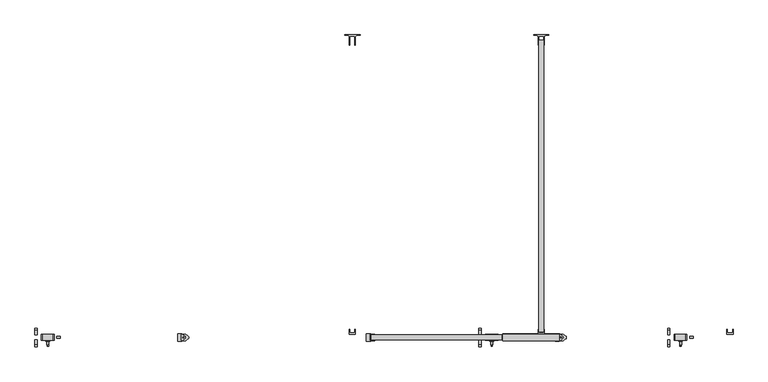
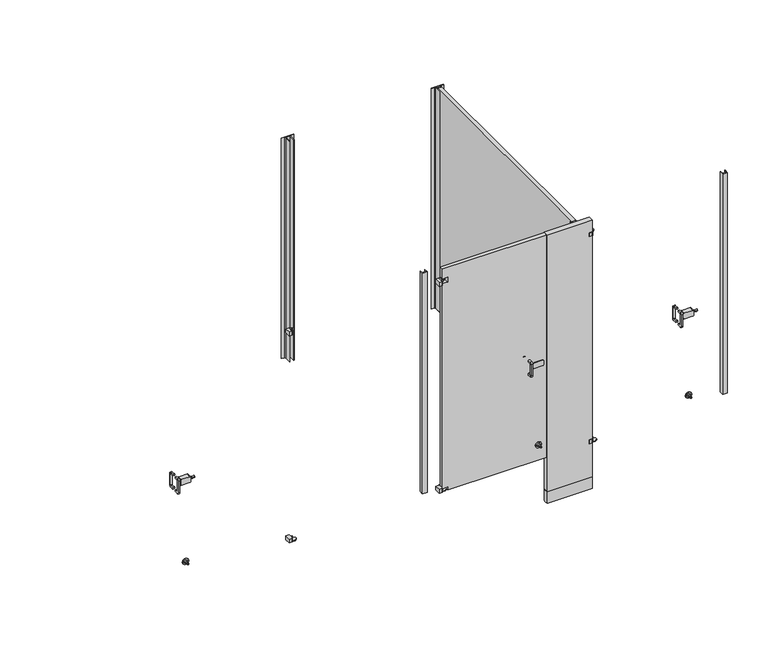
"""IFC4 building model written with IfcOpenShell, lengths in millimetres: proxy geometry, Partition-Floor_Braced-Bradley_Corp-St_Stl-ADA-N_Stalls : ADA (optional) + n Standard Stalls."""

from ifc_helpers import new_model, si_unit, point, frame, frame_2d, origin, origin_with_axes, place, context, project, spatial, polyline, circle_curve, ellipse_curve, trimmed, segment, composite_curve, outline, extrude, source, transform, mapped, element, save
from ifc_brep_helpers import plane_surface, cylinder_surface, revolved_surface, advanced_brep


def specialty_equipment_3ab3950b(model_context):
    return source(origin(), model_context, "Body", "SolidModel", [
        extrude(outline(composite_curve([segment(trimmed(circle_curve(frame_2d((-1469.3891724, 977.9)), 10.16), [point((-1469.3891724, 988.06))], [point((-1459.2291724, 977.9))], False, "CARTESIAN"), True, "CONTINUOUS"), segment(polyline([(-1459.2291724, 977.9), (-1459.2291724, 901.7)]), True, "CONTINUOUS"), segment(trimmed(circle_curve(frame_2d((-1469.3891724, 901.7)), 10.16), [point((-1459.2291724, 901.7))], [point((-1469.3891724, 891.54))], False, "CARTESIAN"), True, "CONTINUOUS"), segment(polyline([(-1469.3891724, 891.54), (-1492.2491724, 891.54), (-1492.2491724, 901.7), (-1469.3891724, 901.7)]), True, "CONTINUOUS"), segment(trimmed(circle_curve(frame_2d((-1469.3891724, 904.24)), 2.54), [point((-1469.3891724, 901.7))], [point((-1466.8491724, 904.24))], True, "CARTESIAN"), True, "CONTINUOUS"), segment(polyline([(-1466.8491724, 904.24), (-1466.8491724, 975.36)]), True, "CONTINUOUS"), segment(trimmed(circle_curve(frame_2d((-1469.3891724, 975.36)), 2.54), [point((-1466.8491724, 975.36))], [point((-1469.3891724, 977.9))], True, "CARTESIAN"), True, "CONTINUOUS"), segment(polyline([(-1469.3891724, 977.9), (-1492.2491724, 977.9), (-1492.2491724, 988.06), (-1469.3891724, 988.06)]), True, "CONTINUOUS")], self_intersect=False)), frame((1086.5228738, 0.0, 0.0), z_axis=(1.0, 0.0, 0.0), x_axis=(0.0, 1.0, 0.0)), (0.0, 0.0, 1.0), 11.4113578),
        extrude(outline(composite_curve([segment(polyline([(-1540.51, 988.06), (-1517.65, 988.06), (-1517.65, 977.9), (-1540.51, 977.9)]), True, "CONTINUOUS"), segment(trimmed(circle_curve(frame_2d((-1540.51, 975.36)), 2.54), [point((-1540.51, 977.9))], [point((-1543.05, 975.36))], True, "CARTESIAN"), True, "CONTINUOUS"), segment(polyline([(-1543.05, 975.36), (-1543.05, 904.24)]), True, "CONTINUOUS"), segment(trimmed(circle_curve(frame_2d((-1540.51, 904.24)), 2.54), [point((-1543.05, 904.24))], [point((-1540.51, 901.7))], True, "CARTESIAN"), True, "CONTINUOUS"), segment(polyline([(-1540.51, 901.7), (-1517.65, 901.7), (-1517.65, 891.54), (-1540.51, 891.54)]), True, "CONTINUOUS"), segment(trimmed(circle_curve(frame_2d((-1540.51, 901.7)), 10.16), [point((-1540.51, 891.54))], [point((-1550.67, 901.7))], False, "CARTESIAN"), True, "CONTINUOUS"), segment(polyline([(-1550.67, 901.7), (-1550.67, 977.9)]), True, "CONTINUOUS"), segment(trimmed(circle_curve(frame_2d((-1540.51, 977.9)), 10.16), [point((-1550.67, 977.9))], [point((-1540.51, 988.06))], False, "CARTESIAN"), True, "CONTINUOUS")], self_intersect=False)), frame((1086.5228738, 0.0, 0.0), z_axis=(1.0, 0.0, 0.0), x_axis=(0.0, 1.0, 0.0)), (0.0, 0.0, 1.0), 11.4113578),
        extrude(outline(composite_curve([segment(trimmed(circle_curve(frame_2d((406.4, 1150.9250547)), 3.4532283), [point((402.9467717, 1150.9250547))], [point((409.8532283, 1150.9250547))], False, "CARTESIAN"), True, "CONTINUOUS"), segment(trimmed(circle_curve(frame_2d((406.4, 1150.9250547)), 3.4532283), [point((409.8532283, 1150.9250547))], [point((402.9467717, 1150.9250547))], False, "CARTESIAN"), True, "CONTINUOUS")], self_intersect=False)), frame((0.0, -1548.13, 0.0), z_axis=(0.0, 1.0, 0.0), x_axis=(0.0, 0.0, 1.0)), (0.0, 0.0, 1.0), 7.62),
        advanced_brep(
        [(1150.9250547, -1517.65, 406.4), (1131.8750547, -1517.65, 406.4), (1169.9750547, -1517.65, 406.4), (1156.0050547, -1540.51, 406.4), (1145.8450547, -1540.51, 406.4), (1150.9250547, -1540.51, 406.4), (1156.0050547, -1525.27, 406.4), (1145.8450547, -1525.27, 406.4), (1161.0850547, -1520.19, 406.4), (1140.7650547, -1520.19, 406.4), (1169.9750547, -1520.19, 406.4), (1131.8750547, -1520.19, 406.4)],
        [
            (0, 1),
            (1, 2, circle_curve(frame((1150.9250547, -1517.65, 406.4), z_axis=(0.0, 1.0, 0.0), x_axis=(-1.0, 0.0, 0.0)), 19.05)),
            (2, 0),
            (2, 1, circle_curve(frame((1150.9250547, -1517.65, 406.4), z_axis=(0.0, 1.0, 0.0), x_axis=(-1.0, 0.0, 0.0)), 19.05)),
            (3, 4, circle_curve(frame((1150.9250547, -1540.51, 406.4), z_axis=(0.0, -1.0, 0.0), x_axis=(-1.0, 0.0, 0.0)), 5.08)),
            (4, 5),
            (5, 3),
            (4, 3, circle_curve(frame((1150.9250547, -1540.51, 406.4), z_axis=(0.0, -1.0, 0.0), x_axis=(-1.0, 0.0, 0.0)), 5.08)),
            (6, 7, circle_curve(frame((1150.9250547, -1525.27, 406.4), z_axis=(0.0, -1.0, 0.0), x_axis=(-1.0, 0.0, 0.0)), 5.08)),
            (7, 4),
            (3, 6),
            (7, 6, circle_curve(frame((1150.9250547, -1525.27, 406.4), z_axis=(0.0, -1.0, 0.0), x_axis=(-1.0, 0.0, 0.0)), 5.08)),
            (8, 9, circle_curve(frame((1150.9250547, -1520.19, 406.4), z_axis=(0.0, -1.0, 0.0), x_axis=(-1.0, 0.0, 0.0)), 10.16)),
            (9, 7, circle_curve(frame((1145.8450547, -1520.19, 406.4), z_axis=(0.0, 0.0, 1.0), x_axis=(0.0, -1.0, 0.0)), 5.08)),
            (6, 8, circle_curve(frame((1156.0050547, -1520.19, 406.4), z_axis=(0.0, 0.0, 1.0), x_axis=(0.0, -1.0, 0.0)), 5.08)),
            (9, 8, circle_curve(frame((1150.9250547, -1520.19, 406.4), z_axis=(0.0, -1.0, 0.0), x_axis=(-1.0, 0.0, 0.0)), 10.16)),
            (10, 11, circle_curve(frame((1150.9250547, -1520.19, 406.4), z_axis=(0.0, -1.0, 0.0), x_axis=(-1.0, 0.0, 0.0)), 19.05)),
            (11, 9),
            (8, 10),
            (11, 10, circle_curve(frame((1150.9250547, -1520.19, 406.4), z_axis=(0.0, -1.0, 0.0), x_axis=(-1.0, 0.0, 0.0)), 19.05)),
            (1, 11),
            (10, 2),
        ],
        [
            plane_surface(frame((1150.9250547, -1517.65, 406.4), z_axis=(0.0, 1.0, 0.0), x_axis=(-1.0, 0.0, 0.0))),
            plane_surface(frame((1150.9250547, -1540.51, 406.4), z_axis=(0.0, -1.0, 0.0), x_axis=(-1.0, 0.0, 0.0))),
            cylinder_surface(frame((1150.9250547, -1561.6297247, 406.4), z_axis=(0.0, 1.0, 0.0), x_axis=(-1.0, 0.0, 0.0)), 5.08),
            revolved_surface(trimmed(ellipse_curve(frame((1145.8450547, -1520.19, 406.4), z_axis=(0.0, 0.0, -1.0), x_axis=(0.0, -1.0, 0.0)), 5.08, 5.08), [point((1145.8450547, -1525.27, 406.4))], [point((1140.7650547, -1520.19, 406.4))], True, "CARTESIAN"), (1150.9250547, -1561.6297247, 406.4), (0.0, 1.0, 0.0)),
            plane_surface(frame((1150.9250547, -1520.19, 406.4), z_axis=(0.0, -1.0, 0.0), x_axis=(-1.0, 0.0, 0.0))),
            cylinder_surface(frame((1150.9250547, -1561.6297247, 406.4), z_axis=(0.0, 1.0, 0.0), x_axis=(-1.0, 0.0, 0.0)), 19.05),
        ],
        [
            (0, [[1, 2, 3]]),
            (0, [[-3, 4, -1]]),
            (1, [[5, 6, 7]]),
            (1, [[8, -7, -6]]),
            (2, [[9, 10, -5, 11]]),
            (2, [[12, -11, -8, -10]]),
            (3, [[13, 14, -9, 15]]),
            (3, [[16, -15, -12, -14]]),
            (4, [[17, 18, -13, 19]]),
            (4, [[20, -19, -16, -18]]),
            (5, [[-2, 21, -17, 22]]),
            (5, [[-4, -22, -20, -21]]),
        ],
    ),
        advanced_brep(
        [(1195.3750547, -1499.87, 939.8), (1195.3750547, -1510.03, 939.8), (1212.8502547, -1510.03, 939.8), (1212.8502547, -1499.87, 939.8), (1195.3750547, -1504.95, 939.8), (1212.8502547, -1504.95, 939.8)],
        [
            (0, 1, circle_curve(frame((1195.3750547, -1504.95, 939.8), z_axis=(1.0, 0.0, 0.0), x_axis=(0.0, -1.0, 0.0)), 5.08)),
            (1, 2),
            (2, 3, circle_curve(frame((1212.8502547, -1504.95, 939.8), z_axis=(-1.0, 0.0, 0.0), x_axis=(0.0, -1.0, 0.0)), 5.08)),
            (3, 0),
            (1, 0, circle_curve(frame((1195.3750547, -1504.95, 939.8), z_axis=(1.0, 0.0, 0.0), x_axis=(0.0, -1.0, 0.0)), 5.08)),
            (3, 2, circle_curve(frame((1212.8502547, -1504.95, 939.8), z_axis=(-1.0, 0.0, 0.0), x_axis=(0.0, -1.0, 0.0)), 5.08)),
            (4, 1),
            (0, 4),
            (2, 5),
            (5, 3),
        ],
        [
            cylinder_surface(frame((1212.8502547, -1504.95, 939.8), z_axis=(-1.0, 0.0, 0.0), x_axis=(0.0, -1.0, 0.0)), 5.08),
            plane_surface(frame((1195.3750547, -1504.95, 939.8), z_axis=(-1.0, 0.0, 0.0), x_axis=(0.0, -1.0, 0.0))),
            plane_surface(frame((1212.8502547, -1504.95, 939.8), z_axis=(1.0, 0.0, 0.0), x_axis=(0.0, -1.0, 0.0))),
        ],
        [
            (0, [[1, 2, 3, 4]]),
            (0, [[5, -4, 6, -2]]),
            (1, [[7, -1, 8]]),
            (1, [[-8, -5, -7]]),
            (2, [[-3, 9, 10]]),
            (2, [[-6, -10, -9]]),
        ],
    ),
        extrude(outline(composite_curve([segment(trimmed(circle_curve(frame_2d((926.0058992, 1124.4309539)), 5.2558992), [point((926.0058992, 1119.1750547))], [point((920.75, 1124.4309539))], False, "CARTESIAN"), True, "CONTINUOUS"), segment(polyline([(920.75, 1124.4309539), (920.75, 1177.4191555)]), True, "CONTINUOUS"), segment(trimmed(circle_curve(frame_2d((926.0058992, 1177.4191555)), 5.2558992), [point((920.75, 1177.4191555))], [point((926.0058992, 1182.6750547))], False, "CARTESIAN"), True, "CONTINUOUS"), segment(polyline([(926.0058992, 1182.6750547), (953.5941008, 1182.6750547)]), True, "CONTINUOUS"), segment(trimmed(circle_curve(frame_2d((953.5941008, 1177.4191555)), 5.2558992), [point((953.5941008, 1182.6750547))], [point((958.85, 1177.4191555))], False, "CARTESIAN"), True, "CONTINUOUS"), segment(polyline([(958.85, 1177.4191555), (958.85, 1124.4309539)]), True, "CONTINUOUS"), segment(trimmed(circle_curve(frame_2d((953.5941008, 1124.4309539)), 5.2558992), [point((958.85, 1124.4309539))], [point((953.5941008, 1119.1750547))], False, "CARTESIAN"), True, "CONTINUOUS"), segment(polyline([(953.5941008, 1119.1750547), (926.0058992, 1119.1750547)]), True, "CONTINUOUS")], self_intersect=False)), frame((0.0, -1519.555, 0.0), z_axis=(0.0, 1.0, 0.0), x_axis=(0.0, 0.0, 1.0)), (0.0, 0.0, 1.0), 29.21),
        extrude(outline(composite_curve([segment(trimmed(circle_curve(frame_2d((-1469.3891724, 977.9)), 10.16), [point((-1469.3891724, 988.06))], [point((-1459.2291724, 977.9))], False, "CARTESIAN"), True, "CONTINUOUS"), segment(polyline([(-1459.2291724, 977.9), (-1459.2291724, 901.7)]), True, "CONTINUOUS"), segment(trimmed(circle_curve(frame_2d((-1469.3891724, 901.7)), 10.16), [point((-1459.2291724, 901.7))], [point((-1469.3891724, 891.54))], False, "CARTESIAN"), True, "CONTINUOUS"), segment(polyline([(-1469.3891724, 891.54), (-1492.2491724, 891.54), (-1492.2491724, 901.7), (-1469.3891724, 901.7)]), True, "CONTINUOUS"), segment(trimmed(circle_curve(frame_2d((-1469.3891724, 904.24)), 2.54), [point((-1469.3891724, 901.7))], [point((-1466.8491724, 904.24))], True, "CARTESIAN"), True, "CONTINUOUS"), segment(polyline([(-1466.8491724, 904.24), (-1466.8491724, 975.36)]), True, "CONTINUOUS"), segment(trimmed(circle_curve(frame_2d((-1469.3891724, 975.36)), 2.54), [point((-1466.8491724, 975.36))], [point((-1469.3891724, 977.9))], True, "CARTESIAN"), True, "CONTINUOUS"), segment(polyline([(-1469.3891724, 977.9), (-1492.2491724, 977.9), (-1492.2491724, 988.06), (-1469.3891724, 988.06)]), True, "CONTINUOUS")], self_intersect=False)), frame((4236.1228738, 0.0, 0.0), z_axis=(1.0, 0.0, 0.0), x_axis=(0.0, 1.0, 0.0)), (0.0, 0.0, 1.0), 11.4113578),
        extrude(outline(composite_curve([segment(polyline([(-1540.51, 988.06), (-1517.65, 988.06), (-1517.65, 977.9), (-1540.51, 977.9)]), True, "CONTINUOUS"), segment(trimmed(circle_curve(frame_2d((-1540.51, 975.36)), 2.54), [point((-1540.51, 977.9))], [point((-1543.05, 975.36))], True, "CARTESIAN"), True, "CONTINUOUS"), segment(polyline([(-1543.05, 975.36), (-1543.05, 904.24)]), True, "CONTINUOUS"), segment(trimmed(circle_curve(frame_2d((-1540.51, 904.24)), 2.54), [point((-1543.05, 904.24))], [point((-1540.51, 901.7))], True, "CARTESIAN"), True, "CONTINUOUS"), segment(polyline([(-1540.51, 901.7), (-1517.65, 901.7), (-1517.65, 891.54), (-1540.51, 891.54)]), True, "CONTINUOUS"), segment(trimmed(circle_curve(frame_2d((-1540.51, 901.7)), 10.16), [point((-1540.51, 891.54))], [point((-1550.67, 901.7))], False, "CARTESIAN"), True, "CONTINUOUS"), segment(polyline([(-1550.67, 901.7), (-1550.67, 977.9)]), True, "CONTINUOUS"), segment(trimmed(circle_curve(frame_2d((-1540.51, 977.9)), 10.16), [point((-1550.67, 977.9))], [point((-1540.51, 988.06))], False, "CARTESIAN"), True, "CONTINUOUS")], self_intersect=False)), frame((4236.1228738, 0.0, 0.0), z_axis=(1.0, 0.0, 0.0), x_axis=(0.0, 1.0, 0.0)), (0.0, 0.0, 1.0), 11.4113578),
        extrude(outline(composite_curve([segment(trimmed(circle_curve(frame_2d((406.4, 4300.5250547)), 3.4532283), [point((402.9467717, 4300.5250547))], [point((409.8532283, 4300.5250547))], False, "CARTESIAN"), True, "CONTINUOUS"), segment(trimmed(circle_curve(frame_2d((406.4, 4300.5250547)), 3.4532283), [point((409.8532283, 4300.5250547))], [point((402.9467717, 4300.5250547))], False, "CARTESIAN"), True, "CONTINUOUS")], self_intersect=False)), frame((0.0, -1548.13, 0.0), z_axis=(0.0, 1.0, 0.0), x_axis=(0.0, 0.0, 1.0)), (0.0, 0.0, 1.0), 7.62),
        advanced_brep(
        [(4300.5250547, -1517.65, 406.4), (4281.4750547, -1517.65, 406.4), (4319.5750547, -1517.65, 406.4), (4305.6050547, -1540.51, 406.4), (4295.4450547, -1540.51, 406.4), (4300.5250547, -1540.51, 406.4), (4305.6050547, -1525.27, 406.4), (4295.4450547, -1525.27, 406.4), (4310.6850547, -1520.19, 406.4), (4290.3650547, -1520.19, 406.4), (4319.5750547, -1520.19, 406.4), (4281.4750547, -1520.19, 406.4)],
        [
            (0, 1),
            (1, 2, circle_curve(frame((4300.5250547, -1517.65, 406.4), z_axis=(0.0, 1.0, 0.0), x_axis=(-1.0, 0.0, 0.0)), 19.05)),
            (2, 0),
            (2, 1, circle_curve(frame((4300.5250547, -1517.65, 406.4), z_axis=(0.0, 1.0, 0.0), x_axis=(-1.0, 0.0, 0.0)), 19.05)),
            (3, 4, circle_curve(frame((4300.5250547, -1540.51, 406.4), z_axis=(0.0, -1.0, 0.0), x_axis=(-1.0, 0.0, 0.0)), 5.08)),
            (4, 5),
            (5, 3),
            (4, 3, circle_curve(frame((4300.5250547, -1540.51, 406.4), z_axis=(0.0, -1.0, 0.0), x_axis=(-1.0, 0.0, 0.0)), 5.08)),
            (6, 7, circle_curve(frame((4300.5250547, -1525.27, 406.4), z_axis=(0.0, -1.0, 0.0), x_axis=(-1.0, 0.0, 0.0)), 5.08)),
            (7, 4),
            (3, 6),
            (7, 6, circle_curve(frame((4300.5250547, -1525.27, 406.4), z_axis=(0.0, -1.0, 0.0), x_axis=(-1.0, 0.0, 0.0)), 5.08)),
            (8, 9, circle_curve(frame((4300.5250547, -1520.19, 406.4), z_axis=(0.0, -1.0, 0.0), x_axis=(-1.0, 0.0, 0.0)), 10.16)),
            (9, 7, circle_curve(frame((4295.4450547, -1520.19, 406.4), z_axis=(0.0, 0.0, 1.0), x_axis=(0.0, -1.0, 0.0)), 5.08)),
            (6, 8, circle_curve(frame((4305.6050547, -1520.19, 406.4), z_axis=(0.0, 0.0, 1.0), x_axis=(0.0, -1.0, 0.0)), 5.08)),
            (9, 8, circle_curve(frame((4300.5250547, -1520.19, 406.4), z_axis=(0.0, -1.0, 0.0), x_axis=(-1.0, 0.0, 0.0)), 10.16)),
            (10, 11, circle_curve(frame((4300.5250547, -1520.19, 406.4), z_axis=(0.0, -1.0, 0.0), x_axis=(-1.0, 0.0, 0.0)), 19.05)),
            (11, 9),
            (8, 10),
            (11, 10, circle_curve(frame((4300.5250547, -1520.19, 406.4), z_axis=(0.0, -1.0, 0.0), x_axis=(-1.0, 0.0, 0.0)), 19.05)),
            (1, 11),
            (10, 2),
        ],
        [
            plane_surface(frame((4300.5250547, -1517.65, 406.4), z_axis=(0.0, 1.0, 0.0), x_axis=(-1.0, 0.0, 0.0))),
            plane_surface(frame((4300.5250547, -1540.51, 406.4), z_axis=(0.0, -1.0, 0.0), x_axis=(-1.0, 0.0, 0.0))),
            cylinder_surface(frame((4300.5250547, -1561.6297247, 406.4), z_axis=(0.0, 1.0, 0.0), x_axis=(-1.0, 0.0, 0.0)), 5.08),
            revolved_surface(trimmed(ellipse_curve(frame((4295.4450547, -1520.19, 406.4), z_axis=(0.0, 0.0, -1.0), x_axis=(0.0, -1.0, 0.0)), 5.08, 5.08), [point((4295.4450547, -1525.27, 406.4))], [point((4290.3650547, -1520.19, 406.4))], True, "CARTESIAN"), (4300.5250547, -1561.6297247, 406.4), (0.0, 1.0, 0.0)),
            plane_surface(frame((4300.5250547, -1520.19, 406.4), z_axis=(0.0, -1.0, 0.0), x_axis=(-1.0, 0.0, 0.0))),
            cylinder_surface(frame((4300.5250547, -1561.6297247, 406.4), z_axis=(0.0, 1.0, 0.0), x_axis=(-1.0, 0.0, 0.0)), 19.05),
        ],
        [
            (0, [[1, 2, 3]]),
            (0, [[-3, 4, -1]]),
            (1, [[5, 6, 7]]),
            (1, [[8, -7, -6]]),
            (2, [[9, 10, -5, 11]]),
            (2, [[12, -11, -8, -10]]),
            (3, [[13, 14, -9, 15]]),
            (3, [[16, -15, -12, -14]]),
            (4, [[17, 18, -13, 19]]),
            (4, [[20, -19, -16, -18]]),
            (5, [[-2, 21, -17, 22]]),
            (5, [[-4, -22, -20, -21]]),
        ],
    ),
        advanced_brep(
        [(4344.9750547, -1499.87, 939.8), (4344.9750547, -1510.03, 939.8), (4362.4502547, -1510.03, 939.8), (4362.4502547, -1499.87, 939.8), (4344.9750547, -1504.95, 939.8), (4362.4502547, -1504.95, 939.8)],
        [
            (0, 1, circle_curve(frame((4344.9750547, -1504.95, 939.8), z_axis=(1.0, 0.0, 0.0), x_axis=(0.0, -1.0, 0.0)), 5.08)),
            (1, 2),
            (2, 3, circle_curve(frame((4362.4502547, -1504.95, 939.8), z_axis=(-1.0, 0.0, 0.0), x_axis=(0.0, -1.0, 0.0)), 5.08)),
            (3, 0),
            (1, 0, circle_curve(frame((4344.9750547, -1504.95, 939.8), z_axis=(1.0, 0.0, 0.0), x_axis=(0.0, -1.0, 0.0)), 5.08)),
            (3, 2, circle_curve(frame((4362.4502547, -1504.95, 939.8), z_axis=(-1.0, 0.0, 0.0), x_axis=(0.0, -1.0, 0.0)), 5.08)),
            (4, 1),
            (0, 4),
            (2, 5),
            (5, 3),
        ],
        [
            cylinder_surface(frame((4362.4502547, -1504.95, 939.8), z_axis=(-1.0, 0.0, 0.0), x_axis=(0.0, -1.0, 0.0)), 5.08),
            plane_surface(frame((4344.9750547, -1504.95, 939.8), z_axis=(-1.0, 0.0, 0.0), x_axis=(0.0, -1.0, 0.0))),
            plane_surface(frame((4362.4502547, -1504.95, 939.8), z_axis=(1.0, 0.0, 0.0), x_axis=(0.0, -1.0, 0.0))),
        ],
        [
            (0, [[1, 2, 3, 4]]),
            (0, [[5, -4, 6, -2]]),
            (1, [[7, -1, 8]]),
            (1, [[-8, -5, -7]]),
            (2, [[-3, 9, 10]]),
            (2, [[-6, -10, -9]]),
        ],
    ),
        extrude(outline(composite_curve([segment(trimmed(circle_curve(frame_2d((926.0058992, 4274.0309539)), 5.2558992), [point((926.0058992, 4268.7750547))], [point((920.75, 4274.0309539))], False, "CARTESIAN"), True, "CONTINUOUS"), segment(polyline([(920.75, 4274.0309539), (920.75, 4327.0191555)]), True, "CONTINUOUS"), segment(trimmed(circle_curve(frame_2d((926.0058992, 4327.0191555)), 5.2558992), [point((920.75, 4327.0191555))], [point((926.0058992, 4332.2750547))], False, "CARTESIAN"), True, "CONTINUOUS"), segment(polyline([(926.0058992, 4332.2750547), (953.5941008, 4332.2750547)]), True, "CONTINUOUS"), segment(trimmed(circle_curve(frame_2d((953.5941008, 4327.0191555)), 5.2558992), [point((953.5941008, 4332.2750547))], [point((958.85, 4327.0191555))], False, "CARTESIAN"), True, "CONTINUOUS"), segment(polyline([(958.85, 4327.0191555), (958.85, 4274.0309539)]), True, "CONTINUOUS"), segment(trimmed(circle_curve(frame_2d((953.5941008, 4274.0309539)), 5.2558992), [point((958.85, 4274.0309539))], [point((953.5941008, 4268.7750547))], False, "CARTESIAN"), True, "CONTINUOUS"), segment(polyline([(953.5941008, 4268.7750547), (926.0058992, 4268.7750547)]), True, "CONTINUOUS")], self_intersect=False)), frame((0.0, -1519.555, 0.0), z_axis=(0.0, 1.0, 0.0), x_axis=(0.0, 0.0, 1.0)), (0.0, 0.0, 1.0), 29.21),
        extrude(outline(polyline([(3591.5602547, -1489.075), (3591.5602547, -1463.675), (3594.1002547, -1463.675), (3594.1002547, -1482.1271812), (3619.5002547, -1482.1271812), (3619.5002547, -1463.675), (3622.0402547, -1463.675), (3622.0402547, -1489.075), (3591.5602547, -1489.075)])), frame((0.0, 0.0, 311.15), z_axis=(0.0, 0.0, 1.0), x_axis=(1.0, 0.0, 0.0)), (0.0, 0.0, 1.0), 1460.5),
        extrude(outline(composite_curve([segment(polyline([(3644.9002547, 3.175), (3644.9002547, 0.635), (3628.3902547, 0.635)]), True, "CONTINUOUS"), segment(trimmed(circle_curve(frame_2d((3628.3902547, -5.715)), 6.35), [point((3628.3902547, 0.635))], [point((3622.0402547, -5.715))], True, "CARTESIAN"), True, "CONTINUOUS"), segment(polyline([(3622.0402547, -5.715), (3622.0402547, -47.625), (3619.5002547, -47.625), (3619.5002547, -3.7728188), (3594.1002547, -3.7728188), (3594.1002547, -47.625), (3591.5602547, -47.625), (3591.5602547, -5.715)]), True, "CONTINUOUS"), segment(trimmed(circle_curve(frame_2d((3585.2102547, -5.715)), 6.35), [point((3591.5602547, -5.715))], [point((3585.2102547, 0.635))], True, "CARTESIAN"), True, "CONTINUOUS"), segment(polyline([(3585.2102547, 0.635), (3568.7002547, 0.635), (3568.7002547, 3.175), (3644.9002547, 3.175)]), True, "CONTINUOUS")], self_intersect=False)), frame((0.0, 0.0, 311.15), z_axis=(0.0, 0.0, 1.0), x_axis=(1.0, 0.0, 0.0)), (0.0, 0.0, 1.0), 1460.5),
        extrude(outline(composite_curve([segment(trimmed(circle_curve(frame_2d((2765.7554547, -1504.95)), 2.54), [point((2765.7554547, -1507.49))], [point((2765.7554547, -1502.41))], False, "CARTESIAN"), True, "CONTINUOUS"), segment(trimmed(circle_curve(frame_2d((2765.7554547, -1504.95)), 2.54), [point((2765.7554547, -1502.41))], [point((2765.7554547, -1507.49))], False, "CARTESIAN"), True, "CONTINUOUS")], self_intersect=False)), frame((0.0, 0.0, 304.8), z_axis=(0.0, 0.0, 1.0), x_axis=(1.0, 0.0, 0.0)), (0.0, 0.0, 1.0), 25.4),
        extrude(outline(composite_curve([segment(polyline([(2755.9002547, -1489.71), (2777.4902547, -1489.075), (2787.6502547, -1497.33)]), True, "CONTINUOUS"), segment(trimmed(circle_curve(frame_2d((2783.8402547, -1504.95)), 8.519419), [point((2787.6502547, -1497.33))], [point((2787.6502547, -1512.57))], False, "CARTESIAN"), True, "CONTINUOUS"), segment(polyline([(2787.6502547, -1512.57), (2777.4902547, -1520.825), (2755.9002547, -1520.19), (2755.9002547, -1489.71)]), True, "CONTINUOUS")], self_intersect=False)), frame((0.0, 0.0, 304.8), z_axis=(0.0, 0.0, 1.0), x_axis=(1.0, 0.0, 0.0)), (0.0, 0.0, 1.0), 3.81),
        extrude(outline(composite_curve([segment(polyline([(2736.8502547, -1486.535), (2755.9002547, -1486.535)]), True, "CONTINUOUS"), segment(trimmed(circle_curve(frame_2d((2755.9002547, -1489.075)), 2.54), [point((2755.9002547, -1486.535))], [point((2758.4402547, -1489.075))], False, "CARTESIAN"), True, "CONTINUOUS"), segment(trimmed(circle_curve(frame_2d((2650.6397496, -1504.95)), 108.9631338), [point((2758.4402547, -1489.075))], [point((2758.4402547, -1520.825))], False, "CARTESIAN"), True, "CONTINUOUS"), segment(trimmed(circle_curve(frame_2d((2755.9002547, -1520.825)), 2.54), [point((2758.4402547, -1520.825))], [point((2755.9002547, -1523.365))], False, "CARTESIAN"), True, "CONTINUOUS"), segment(polyline([(2755.9002547, -1523.365), (2736.8502547, -1523.365), (2736.8502547, -1486.535)]), True, "CONTINUOUS")], self_intersect=False)), frame((0.0, 0.0, 304.8), z_axis=(0.0, 0.0, 1.0), x_axis=(1.0, 0.0, 0.0)), (0.0, 0.0, 1.0), 25.4),
        extrude(outline(composite_curve([segment(trimmed(circle_curve(frame_2d((2765.7554547, -1504.95)), 2.54), [point((2765.7554547, -1507.49))], [point((2765.7554547, -1502.41))], False, "CARTESIAN"), True, "CONTINUOUS"), segment(trimmed(circle_curve(frame_2d((2765.7554547, -1504.95)), 2.54), [point((2765.7554547, -1502.41))], [point((2765.7554547, -1507.49))], False, "CARTESIAN"), True, "CONTINUOUS")], self_intersect=False)), frame((0.0, 0.0, 1676.4), z_axis=(0.0, 0.0, 1.0), x_axis=(1.0, 0.0, 0.0)), (0.0, 0.0, 1.0), 25.4),
        extrude(outline(composite_curve([segment(polyline([(2760.6754547, -1520.825), (2755.9002547, -1520.19), (2755.9002547, -1489.71), (2760.6754547, -1489.075), (2770.8354547, -1497.33)]), True, "CONTINUOUS"), segment(trimmed(circle_curve(frame_2d((2767.0254547, -1504.95)), 8.519419), [point((2770.8354547, -1497.33))], [point((2770.8354547, -1512.57))], False, "CARTESIAN"), True, "CONTINUOUS"), segment(polyline([(2770.8354547, -1512.57), (2760.6754547, -1520.825)]), True, "CONTINUOUS")], self_intersect=False)), frame((0.0, 0.0, 1697.99), z_axis=(0.0, 0.0, 1.0), x_axis=(1.0, 0.0, 0.0)), (0.0, 0.0, 1.0), 3.81),
        extrude(outline(composite_curve([segment(polyline([(2736.8502547, -1486.535), (2755.9002547, -1486.535)]), True, "CONTINUOUS"), segment(trimmed(circle_curve(frame_2d((2755.9002547, -1489.075)), 2.54), [point((2755.9002547, -1486.535))], [point((2758.4402547, -1489.075))], False, "CARTESIAN"), True, "CONTINUOUS"), segment(trimmed(circle_curve(frame_2d((2650.6397496, -1504.95)), 108.9631338), [point((2758.4402547, -1489.075))], [point((2758.4402547, -1520.825))], False, "CARTESIAN"), True, "CONTINUOUS"), segment(trimmed(circle_curve(frame_2d((2755.9002547, -1520.825)), 2.54), [point((2758.4402547, -1520.825))], [point((2755.9002547, -1523.365))], False, "CARTESIAN"), True, "CONTINUOUS"), segment(polyline([(2755.9002547, -1523.365), (2736.8502547, -1523.365), (2736.8502547, -1486.535)]), True, "CONTINUOUS")], self_intersect=False)), frame((0.0, 0.0, 1676.4), z_axis=(0.0, 0.0, 1.0), x_axis=(1.0, 0.0, 0.0)), (0.0, 0.0, 1.0), 25.4),
        extrude(outline(composite_curve([segment(trimmed(circle_curve(frame_2d((-1469.3891724, 977.9)), 10.16), [point((-1469.3891724, 988.06))], [point((-1459.2291724, 977.9))], False, "CARTESIAN"), True, "CONTINUOUS"), segment(polyline([(-1459.2291724, 977.9), (-1459.2291724, 901.7)]), True, "CONTINUOUS"), segment(trimmed(circle_curve(frame_2d((-1469.3891724, 901.7)), 10.16), [point((-1459.2291724, 901.7))], [point((-1469.3891724, 891.54))], False, "CARTESIAN"), True, "CONTINUOUS"), segment(polyline([(-1469.3891724, 891.54), (-1492.2491724, 891.54), (-1492.2491724, 901.7), (-1469.3891724, 901.7)]), True, "CONTINUOUS"), segment(trimmed(circle_curve(frame_2d((-1469.3891724, 904.24)), 2.54), [point((-1469.3891724, 901.7))], [point((-1466.8491724, 904.24))], True, "CARTESIAN"), True, "CONTINUOUS"), segment(polyline([(-1466.8491724, 904.24), (-1466.8491724, 975.36)]), True, "CONTINUOUS"), segment(trimmed(circle_curve(frame_2d((-1469.3891724, 975.36)), 2.54), [point((-1466.8491724, 975.36))], [point((-1469.3891724, 977.9))], True, "CARTESIAN"), True, "CONTINUOUS"), segment(polyline([(-1469.3891724, 977.9), (-1492.2491724, 977.9), (-1492.2491724, 988.06), (-1469.3891724, 988.06)]), True, "CONTINUOUS")], self_intersect=False)), frame((3296.3228738, 0.0, 0.0), z_axis=(1.0, 0.0, 0.0), x_axis=(0.0, 1.0, 0.0)), (0.0, 0.0, 1.0), 11.4113578),
        extrude(outline(composite_curve([segment(polyline([(-1540.51, 988.06), (-1517.65, 988.06), (-1517.65, 977.9), (-1540.51, 977.9)]), True, "CONTINUOUS"), segment(trimmed(circle_curve(frame_2d((-1540.51, 975.36)), 2.54), [point((-1540.51, 977.9))], [point((-1543.05, 975.36))], True, "CARTESIAN"), True, "CONTINUOUS"), segment(polyline([(-1543.05, 975.36), (-1543.05, 904.24)]), True, "CONTINUOUS"), segment(trimmed(circle_curve(frame_2d((-1540.51, 904.24)), 2.54), [point((-1543.05, 904.24))], [point((-1540.51, 901.7))], True, "CARTESIAN"), True, "CONTINUOUS"), segment(polyline([(-1540.51, 901.7), (-1517.65, 901.7), (-1517.65, 891.54), (-1540.51, 891.54)]), True, "CONTINUOUS"), segment(trimmed(circle_curve(frame_2d((-1540.51, 901.7)), 10.16), [point((-1540.51, 891.54))], [point((-1550.67, 901.7))], False, "CARTESIAN"), True, "CONTINUOUS"), segment(polyline([(-1550.67, 901.7), (-1550.67, 977.9)]), True, "CONTINUOUS"), segment(trimmed(circle_curve(frame_2d((-1540.51, 977.9)), 10.16), [point((-1550.67, 977.9))], [point((-1540.51, 988.06))], False, "CARTESIAN"), True, "CONTINUOUS")], self_intersect=False)), frame((3296.3228738, 0.0, 0.0), z_axis=(1.0, 0.0, 0.0), x_axis=(0.0, 1.0, 0.0)), (0.0, 0.0, 1.0), 11.4113578),
        extrude(outline(composite_curve([segment(trimmed(circle_curve(frame_2d((406.4, 3360.7250547)), 3.4532283), [point((402.9467717, 3360.7250547))], [point((409.8532283, 3360.7250547))], False, "CARTESIAN"), True, "CONTINUOUS"), segment(trimmed(circle_curve(frame_2d((406.4, 3360.7250547)), 3.4532283), [point((409.8532283, 3360.7250547))], [point((402.9467717, 3360.7250547))], False, "CARTESIAN"), True, "CONTINUOUS")], self_intersect=False)), frame((0.0, -1548.13, 0.0), z_axis=(0.0, 1.0, 0.0), x_axis=(0.0, 0.0, 1.0)), (0.0, 0.0, 1.0), 7.62),
        advanced_brep(
        [(3360.7250547, -1517.65, 406.4), (3341.6750547, -1517.65, 406.4), (3379.7750547, -1517.65, 406.4), (3365.8050547, -1540.51, 406.4), (3355.6450547, -1540.51, 406.4), (3360.7250547, -1540.51, 406.4), (3365.8050547, -1525.27, 406.4), (3355.6450547, -1525.27, 406.4), (3370.8850547, -1520.19, 406.4), (3350.5650547, -1520.19, 406.4), (3379.7750547, -1520.19, 406.4), (3341.6750547, -1520.19, 406.4)],
        [
            (0, 1),
            (1, 2, circle_curve(frame((3360.7250547, -1517.65, 406.4), z_axis=(0.0, 1.0, 0.0), x_axis=(-1.0, 0.0, 0.0)), 19.05)),
            (2, 0),
            (2, 1, circle_curve(frame((3360.7250547, -1517.65, 406.4), z_axis=(0.0, 1.0, 0.0), x_axis=(-1.0, 0.0, 0.0)), 19.05)),
            (3, 4, circle_curve(frame((3360.7250547, -1540.51, 406.4), z_axis=(0.0, -1.0, 0.0), x_axis=(-1.0, 0.0, 0.0)), 5.08)),
            (4, 5),
            (5, 3),
            (4, 3, circle_curve(frame((3360.7250547, -1540.51, 406.4), z_axis=(0.0, -1.0, 0.0), x_axis=(-1.0, 0.0, 0.0)), 5.08)),
            (6, 7, circle_curve(frame((3360.7250547, -1525.27, 406.4), z_axis=(0.0, -1.0, 0.0), x_axis=(-1.0, 0.0, 0.0)), 5.08)),
            (7, 4),
            (3, 6),
            (7, 6, circle_curve(frame((3360.7250547, -1525.27, 406.4), z_axis=(0.0, -1.0, 0.0), x_axis=(-1.0, 0.0, 0.0)), 5.08)),
            (8, 9, circle_curve(frame((3360.7250547, -1520.19, 406.4), z_axis=(0.0, -1.0, 0.0), x_axis=(-1.0, 0.0, 0.0)), 10.16)),
            (9, 7, circle_curve(frame((3355.6450547, -1520.19, 406.4), z_axis=(0.0, 0.0, 1.0), x_axis=(0.0, -1.0, 0.0)), 5.08)),
            (6, 8, circle_curve(frame((3365.8050547, -1520.19, 406.4), z_axis=(0.0, 0.0, 1.0), x_axis=(0.0, -1.0, 0.0)), 5.08)),
            (9, 8, circle_curve(frame((3360.7250547, -1520.19, 406.4), z_axis=(0.0, -1.0, 0.0), x_axis=(-1.0, 0.0, 0.0)), 10.16)),
            (10, 11, circle_curve(frame((3360.7250547, -1520.19, 406.4), z_axis=(0.0, -1.0, 0.0), x_axis=(-1.0, 0.0, 0.0)), 19.05)),
            (11, 9),
            (8, 10),
            (11, 10, circle_curve(frame((3360.7250547, -1520.19, 406.4), z_axis=(0.0, -1.0, 0.0), x_axis=(-1.0, 0.0, 0.0)), 19.05)),
            (1, 11),
            (10, 2),
        ],
        [
            plane_surface(frame((3360.7250547, -1517.65, 406.4), z_axis=(0.0, 1.0, 0.0), x_axis=(-1.0, 0.0, 0.0))),
            plane_surface(frame((3360.7250547, -1540.51, 406.4), z_axis=(0.0, -1.0, 0.0), x_axis=(-1.0, 0.0, 0.0))),
            cylinder_surface(frame((3360.7250547, -1561.6297247, 406.4), z_axis=(0.0, 1.0, 0.0), x_axis=(-1.0, 0.0, 0.0)), 5.08),
            revolved_surface(trimmed(ellipse_curve(frame((3355.6450547, -1520.19, 406.4), z_axis=(0.0, 0.0, -1.0), x_axis=(0.0, -1.0, 0.0)), 5.08, 5.08), [point((3355.6450547, -1525.27, 406.4))], [point((3350.5650547, -1520.19, 406.4))], True, "CARTESIAN"), (3360.7250547, -1561.6297247, 406.4), (0.0, 1.0, 0.0)),
            plane_surface(frame((3360.7250547, -1520.19, 406.4), z_axis=(0.0, -1.0, 0.0), x_axis=(-1.0, 0.0, 0.0))),
            cylinder_surface(frame((3360.7250547, -1561.6297247, 406.4), z_axis=(0.0, 1.0, 0.0), x_axis=(-1.0, 0.0, 0.0)), 19.05),
        ],
        [
            (0, [[1, 2, 3]]),
            (0, [[-3, 4, -1]]),
            (1, [[5, 6, 7]]),
            (1, [[8, -7, -6]]),
            (2, [[9, 10, -5, 11]]),
            (2, [[12, -11, -8, -10]]),
            (3, [[13, 14, -9, 15]]),
            (3, [[16, -15, -12, -14]]),
            (4, [[17, 18, -13, 19]]),
            (4, [[20, -19, -16, -18]]),
            (5, [[-2, 21, -17, 22]]),
            (5, [[-4, -22, -20, -21]]),
        ],
    ),
        advanced_brep(
        [(3405.1750547, -1499.87, 939.8), (3405.1750547, -1510.03, 939.8), (3422.6502547, -1510.03, 939.8), (3422.6502547, -1499.87, 939.8), (3405.1750547, -1504.95, 939.8), (3422.6502547, -1504.95, 939.8)],
        [
            (0, 1, circle_curve(frame((3405.1750547, -1504.95, 939.8), z_axis=(1.0, 0.0, 0.0), x_axis=(0.0, -1.0, 0.0)), 5.08)),
            (1, 2),
            (2, 3, circle_curve(frame((3422.6502547, -1504.95, 939.8), z_axis=(-1.0, 0.0, 0.0), x_axis=(0.0, -1.0, 0.0)), 5.08)),
            (3, 0),
            (1, 0, circle_curve(frame((3405.1750547, -1504.95, 939.8), z_axis=(1.0, 0.0, 0.0), x_axis=(0.0, -1.0, 0.0)), 5.08)),
            (3, 2, circle_curve(frame((3422.6502547, -1504.95, 939.8), z_axis=(-1.0, 0.0, 0.0), x_axis=(0.0, -1.0, 0.0)), 5.08)),
            (4, 1),
            (0, 4),
            (2, 5),
            (5, 3),
        ],
        [
            cylinder_surface(frame((3422.6502547, -1504.95, 939.8), z_axis=(-1.0, 0.0, 0.0), x_axis=(0.0, -1.0, 0.0)), 5.08),
            plane_surface(frame((3405.1750547, -1504.95, 939.8), z_axis=(-1.0, 0.0, 0.0), x_axis=(0.0, -1.0, 0.0))),
            plane_surface(frame((3422.6502547, -1504.95, 939.8), z_axis=(1.0, 0.0, 0.0), x_axis=(0.0, -1.0, 0.0))),
        ],
        [
            (0, [[1, 2, 3, 4]]),
            (0, [[5, -4, 6, -2]]),
            (1, [[7, -1, 8]]),
            (1, [[-8, -5, -7]]),
            (2, [[-3, 9, 10]]),
            (2, [[-6, -10, -9]]),
        ],
    ),
        extrude(outline(composite_curve([segment(trimmed(circle_curve(frame_2d((926.0058992, 3334.2309539)), 5.2558992), [point((926.0058992, 3328.9750547))], [point((920.75, 3334.2309539))], False, "CARTESIAN"), True, "CONTINUOUS"), segment(polyline([(920.75, 3334.2309539), (920.75, 3387.2191555)]), True, "CONTINUOUS"), segment(trimmed(circle_curve(frame_2d((926.0058992, 3387.2191555)), 5.2558992), [point((920.75, 3387.2191555))], [point((926.0058992, 3392.4750547))], False, "CARTESIAN"), True, "CONTINUOUS"), segment(polyline([(926.0058992, 3392.4750547), (953.5941008, 3392.4750547)]), True, "CONTINUOUS"), segment(trimmed(circle_curve(frame_2d((953.5941008, 3387.2191555)), 5.2558992), [point((953.5941008, 3392.4750547))], [point((958.85, 3387.2191555))], False, "CARTESIAN"), True, "CONTINUOUS"), segment(polyline([(958.85, 3387.2191555), (958.85, 3334.2309539)]), True, "CONTINUOUS"), segment(trimmed(circle_curve(frame_2d((953.5941008, 3334.2309539)), 5.2558992), [point((958.85, 3334.2309539))], [point((953.5941008, 3328.9750547))], False, "CARTESIAN"), True, "CONTINUOUS"), segment(polyline([(953.5941008, 3328.9750547), (926.0058992, 3328.9750547)]), True, "CONTINUOUS")], self_intersect=False)), frame((0.0, -1519.555, 0.0), z_axis=(0.0, 1.0, 0.0), x_axis=(0.0, 0.0, 1.0)), (0.0, 0.0, 1.0), 29.21),
        extrude(outline(composite_curve([segment(polyline([(3414.7127547, -1487.4875), (3697.2891337, -1487.4875)]), True, "CONTINUOUS"), segment(trimmed(circle_curve(frame_2d((3641.500102, -1504.95)), 58.4581471), [point((3697.2891337, -1487.4875))], [point((3697.2891337, -1522.4125))], False, "CARTESIAN"), True, "CONTINUOUS"), segment(polyline([(3697.2891337, -1522.4125), (3414.7127547, -1522.4125)]), True, "CONTINUOUS"), segment(trimmed(circle_curve(frame_2d((3470.5017864, -1504.95)), 58.4581471), [point((3414.7127547, -1522.4125))], [point((3414.7127547, -1487.4875))], False, "CARTESIAN"), True, "CONTINUOUS")], self_intersect=False)), origin_with_axes(), (0.0, 0.0, 1.0), 76.2),
        extrude(outline(polyline([(3619.5002547, -22.225), (3619.5002547, -1476.375), (3594.1002547, -1476.375), (3594.1002547, -22.225), (3619.5002547, -22.225)])), frame((0.0, 0.0, 304.8), z_axis=(0.0, 0.0, 1.0), x_axis=(1.0, 0.0, 0.0)), (0.0, 0.0, 1.0), 1473.2),
        extrude(outline(polyline([(3416.3002547, -1489.075), (3695.7002547, -1489.075), (3695.7002547, -1520.825), (3416.3002547, -1520.825), (3416.3002547, -1489.075)])), origin_with_axes(), (0.0, 0.0, 1.0), 1778.0),
        extrude(outline(polyline([(1778.0, 3411.5250547), (1778.0, 2760.6754547), (1714.5, 2760.6754547), (1714.5, 2792.4254547), (1682.75, 2792.4254547), (1682.75, 2760.6754547), (323.85, 2760.6754547), (323.85, 2792.4254547), (304.8, 2792.4254547), (304.8, 3411.5250547), (1778.0, 3411.5250547)])), frame((0.0, -1517.65, 0.0), z_axis=(0.0, 1.0, 0.0), x_axis=(0.0, 0.0, 1.0)), (0.0, 0.0, 1.0), 25.4),
        extrude(outline(polyline([(2651.7602547, -1489.075), (2651.7602547, -1463.675), (2654.3002547, -1463.675), (2654.3002547, -1482.1271812), (2679.7002547, -1482.1271812), (2679.7002547, -1463.675), (2682.2402547, -1463.675), (2682.2402547, -1489.075), (2651.7602547, -1489.075)])), frame((0.0, 0.0, 311.15), z_axis=(0.0, 0.0, 1.0), x_axis=(1.0, 0.0, 0.0)), (0.0, 0.0, 1.0), 1460.5),
        extrude(outline(composite_curve([segment(polyline([(2705.1002547, 3.175), (2705.1002547, 0.635), (2688.5902547, 0.635)]), True, "CONTINUOUS"), segment(trimmed(circle_curve(frame_2d((2688.5902547, -5.715)), 6.35), [point((2688.5902547, 0.635))], [point((2682.2402547, -5.715))], True, "CARTESIAN"), True, "CONTINUOUS"), segment(polyline([(2682.2402547, -5.715), (2682.2402547, -47.625), (2679.7002547, -47.625), (2679.7002547, -3.7728188), (2654.3002547, -3.7728188), (2654.3002547, -47.625), (2651.7602547, -47.625), (2651.7602547, -5.715)]), True, "CONTINUOUS"), segment(trimmed(circle_curve(frame_2d((2645.4102547, -5.715)), 6.35), [point((2651.7602547, -5.715))], [point((2645.4102547, 0.635))], True, "CARTESIAN"), True, "CONTINUOUS"), segment(polyline([(2645.4102547, 0.635), (2628.9002547, 0.635), (2628.9002547, 3.175), (2705.1002547, 3.175)]), True, "CONTINUOUS")], self_intersect=False)), frame((0.0, 0.0, 311.15), z_axis=(0.0, 0.0, 1.0), x_axis=(1.0, 0.0, 0.0)), (0.0, 0.0, 1.0), 1460.5),
        extrude(outline(composite_curve([segment(trimmed(circle_curve(frame_2d((1825.9554547, -1504.95)), 2.54), [point((1825.9554547, -1507.49))], [point((1825.9554547, -1502.41))], False, "CARTESIAN"), True, "CONTINUOUS"), segment(trimmed(circle_curve(frame_2d((1825.9554547, -1504.95)), 2.54), [point((1825.9554547, -1502.41))], [point((1825.9554547, -1507.49))], False, "CARTESIAN"), True, "CONTINUOUS")], self_intersect=False)), frame((0.0, 0.0, 304.8), z_axis=(0.0, 0.0, 1.0), x_axis=(1.0, 0.0, 0.0)), (0.0, 0.0, 1.0), 25.4),
        extrude(outline(composite_curve([segment(polyline([(1816.1002547, -1489.71), (1837.6902547, -1489.075), (1847.8502547, -1497.33)]), True, "CONTINUOUS"), segment(trimmed(circle_curve(frame_2d((1844.0402547, -1504.95)), 8.519419), [point((1847.8502547, -1497.33))], [point((1847.8502547, -1512.57))], False, "CARTESIAN"), True, "CONTINUOUS"), segment(polyline([(1847.8502547, -1512.57), (1837.6902547, -1520.825), (1816.1002547, -1520.19), (1816.1002547, -1489.71)]), True, "CONTINUOUS")], self_intersect=False)), frame((0.0, 0.0, 304.8), z_axis=(0.0, 0.0, 1.0), x_axis=(1.0, 0.0, 0.0)), (0.0, 0.0, 1.0), 3.81),
        extrude(outline(composite_curve([segment(polyline([(1797.0502547, -1486.535), (1816.1002547, -1486.535)]), True, "CONTINUOUS"), segment(trimmed(circle_curve(frame_2d((1816.1002547, -1489.075)), 2.54), [point((1816.1002547, -1486.535))], [point((1818.6402547, -1489.075))], False, "CARTESIAN"), True, "CONTINUOUS"), segment(trimmed(circle_curve(frame_2d((1710.8397496, -1504.95)), 108.9631338), [point((1818.6402547, -1489.075))], [point((1818.6402547, -1520.825))], False, "CARTESIAN"), True, "CONTINUOUS"), segment(trimmed(circle_curve(frame_2d((1816.1002547, -1520.825)), 2.54), [point((1818.6402547, -1520.825))], [point((1816.1002547, -1523.365))], False, "CARTESIAN"), True, "CONTINUOUS"), segment(polyline([(1816.1002547, -1523.365), (1797.0502547, -1523.365), (1797.0502547, -1486.535)]), True, "CONTINUOUS")], self_intersect=False)), frame((0.0, 0.0, 304.8), z_axis=(0.0, 0.0, 1.0), x_axis=(1.0, 0.0, 0.0)), (0.0, 0.0, 1.0), 25.4),
        extrude(outline(composite_curve([segment(trimmed(circle_curve(frame_2d((1825.9554547, -1504.95)), 2.54), [point((1825.9554547, -1507.49))], [point((1825.9554547, -1502.41))], False, "CARTESIAN"), True, "CONTINUOUS"), segment(trimmed(circle_curve(frame_2d((1825.9554547, -1504.95)), 2.54), [point((1825.9554547, -1502.41))], [point((1825.9554547, -1507.49))], False, "CARTESIAN"), True, "CONTINUOUS")], self_intersect=False)), frame((0.0, 0.0, 1676.4), z_axis=(0.0, 0.0, 1.0), x_axis=(1.0, 0.0, 0.0)), (0.0, 0.0, 1.0), 25.4),
        extrude(outline(composite_curve([segment(polyline([(1820.8754547, -1520.825), (1816.1002547, -1520.19), (1816.1002547, -1489.71), (1820.8754547, -1489.075), (1831.0354547, -1497.33)]), True, "CONTINUOUS"), segment(trimmed(circle_curve(frame_2d((1827.2254547, -1504.95)), 8.519419), [point((1831.0354547, -1497.33))], [point((1831.0354547, -1512.57))], False, "CARTESIAN"), True, "CONTINUOUS"), segment(polyline([(1831.0354547, -1512.57), (1820.8754547, -1520.825)]), True, "CONTINUOUS")], self_intersect=False)), frame((0.0, 0.0, 1697.99), z_axis=(0.0, 0.0, 1.0), x_axis=(1.0, 0.0, 0.0)), (0.0, 0.0, 1.0), 3.81),
        extrude(outline(composite_curve([segment(polyline([(1797.0502547, -1486.535), (1816.1002547, -1486.535)]), True, "CONTINUOUS"), segment(trimmed(circle_curve(frame_2d((1816.1002547, -1489.075)), 2.54), [point((1816.1002547, -1486.535))], [point((1818.6402547, -1489.075))], False, "CARTESIAN"), True, "CONTINUOUS"), segment(trimmed(circle_curve(frame_2d((1710.8397496, -1504.95)), 108.9631338), [point((1818.6402547, -1489.075))], [point((1818.6402547, -1520.825))], False, "CARTESIAN"), True, "CONTINUOUS"), segment(trimmed(circle_curve(frame_2d((1816.1002547, -1520.825)), 2.54), [point((1818.6402547, -1520.825))], [point((1816.1002547, -1523.365))], False, "CARTESIAN"), True, "CONTINUOUS"), segment(polyline([(1816.1002547, -1523.365), (1797.0502547, -1523.365), (1797.0502547, -1486.535)]), True, "CONTINUOUS")], self_intersect=False)), frame((0.0, 0.0, 1676.4), z_axis=(0.0, 0.0, 1.0), x_axis=(1.0, 0.0, 0.0)), (0.0, 0.0, 1.0), 25.4),
        extrude(outline(composite_curve([segment(trimmed(circle_curve(frame_2d((3705.5554547, -1504.95)), 2.54), [point((3705.5554547, -1507.49))], [point((3705.5554547, -1502.41))], False, "CARTESIAN"), True, "CONTINUOUS"), segment(trimmed(circle_curve(frame_2d((3705.5554547, -1504.95)), 2.54), [point((3705.5554547, -1502.41))], [point((3705.5554547, -1507.49))], False, "CARTESIAN"), True, "CONTINUOUS")], self_intersect=False)), frame((0.0, 0.0, 304.8), z_axis=(0.0, 0.0, 1.0), x_axis=(1.0, 0.0, 0.0)), (0.0, 0.0, 1.0), 25.4),
        extrude(outline(composite_curve([segment(polyline([(3695.7002547, -1489.71), (3717.2902547, -1489.075), (3727.4502547, -1497.33)]), True, "CONTINUOUS"), segment(trimmed(circle_curve(frame_2d((3723.6402547, -1504.95)), 8.519419), [point((3727.4502547, -1497.33))], [point((3727.4502547, -1512.57))], False, "CARTESIAN"), True, "CONTINUOUS"), segment(polyline([(3727.4502547, -1512.57), (3717.2902547, -1520.825), (3695.7002547, -1520.19), (3695.7002547, -1489.71)]), True, "CONTINUOUS")], self_intersect=False)), frame((0.0, 0.0, 304.8), z_axis=(0.0, 0.0, 1.0), x_axis=(1.0, 0.0, 0.0)), (0.0, 0.0, 1.0), 3.81),
        extrude(outline(composite_curve([segment(polyline([(3676.6502547, -1486.535), (3695.7002547, -1486.535)]), True, "CONTINUOUS"), segment(trimmed(circle_curve(frame_2d((3695.7002547, -1489.075)), 2.54), [point((3695.7002547, -1486.535))], [point((3698.2402547, -1489.075))], False, "CARTESIAN"), True, "CONTINUOUS"), segment(trimmed(circle_curve(frame_2d((3590.4397496, -1504.95)), 108.9631338), [point((3698.2402547, -1489.075))], [point((3698.2402547, -1520.825))], False, "CARTESIAN"), True, "CONTINUOUS"), segment(trimmed(circle_curve(frame_2d((3695.7002547, -1520.825)), 2.54), [point((3698.2402547, -1520.825))], [point((3695.7002547, -1523.365))], False, "CARTESIAN"), True, "CONTINUOUS"), segment(polyline([(3695.7002547, -1523.365), (3676.6502547, -1523.365), (3676.6502547, -1486.535)]), True, "CONTINUOUS")], self_intersect=False)), frame((0.0, 0.0, 304.8), z_axis=(0.0, 0.0, 1.0), x_axis=(1.0, 0.0, 0.0)), (0.0, 0.0, 1.0), 25.4),
        extrude(outline(composite_curve([segment(trimmed(circle_curve(frame_2d((3705.5554547, -1504.95)), 2.54), [point((3705.5554547, -1507.49))], [point((3705.5554547, -1502.41))], False, "CARTESIAN"), True, "CONTINUOUS"), segment(trimmed(circle_curve(frame_2d((3705.5554547, -1504.95)), 2.54), [point((3705.5554547, -1502.41))], [point((3705.5554547, -1507.49))], False, "CARTESIAN"), True, "CONTINUOUS")], self_intersect=False)), frame((0.0, 0.0, 1676.4), z_axis=(0.0, 0.0, 1.0), x_axis=(1.0, 0.0, 0.0)), (0.0, 0.0, 1.0), 25.4),
        extrude(outline(composite_curve([segment(polyline([(3700.4754547, -1520.825), (3695.7002547, -1520.19), (3695.7002547, -1489.71), (3700.4754547, -1489.075), (3710.6354547, -1497.33)]), True, "CONTINUOUS"), segment(trimmed(circle_curve(frame_2d((3706.8254547, -1504.95)), 8.519419), [point((3710.6354547, -1497.33))], [point((3710.6354547, -1512.57))], False, "CARTESIAN"), True, "CONTINUOUS"), segment(polyline([(3710.6354547, -1512.57), (3700.4754547, -1520.825)]), True, "CONTINUOUS")], self_intersect=False)), frame((0.0, 0.0, 1697.99), z_axis=(0.0, 0.0, 1.0), x_axis=(1.0, 0.0, 0.0)), (0.0, 0.0, 1.0), 3.81),
        extrude(outline(composite_curve([segment(polyline([(3676.6502547, -1486.535), (3695.7002547, -1486.535)]), True, "CONTINUOUS"), segment(trimmed(circle_curve(frame_2d((3695.7002547, -1489.075)), 2.54), [point((3695.7002547, -1486.535))], [point((3698.2402547, -1489.075))], False, "CARTESIAN"), True, "CONTINUOUS"), segment(trimmed(circle_curve(frame_2d((3590.4397496, -1504.95)), 108.9631338), [point((3698.2402547, -1489.075))], [point((3698.2402547, -1520.825))], False, "CARTESIAN"), True, "CONTINUOUS"), segment(trimmed(circle_curve(frame_2d((3695.7002547, -1520.825)), 2.54), [point((3698.2402547, -1520.825))], [point((3695.7002547, -1523.365))], False, "CARTESIAN"), True, "CONTINUOUS"), segment(polyline([(3695.7002547, -1523.365), (3676.6502547, -1523.365), (3676.6502547, -1486.535)]), True, "CONTINUOUS")], self_intersect=False)), frame((0.0, 0.0, 1676.4), z_axis=(0.0, 0.0, 1.0), x_axis=(1.0, 0.0, 0.0)), (0.0, 0.0, 1.0), 25.4),
        extrude(outline(polyline([(4531.3602547, -1489.075), (4531.3602547, -1463.675), (4533.9002547, -1463.675), (4533.9002547, -1482.1271812), (4559.3002547, -1482.1271812), (4559.3002547, -1463.675), (4561.8402547, -1463.675), (4561.8402547, -1489.075), (4531.3602547, -1489.075)])), frame((0.0, 0.0, 311.15), z_axis=(0.0, 0.0, 1.0), x_axis=(1.0, 0.0, 0.0)), (0.0, 0.0, 1.0), 1460.5),
    ])


if __name__ == "__main__":
    model = new_model("IFC4")
    model_context = context("Model", 3, world=origin())
    ifc_project = project(units=[si_unit("LENGTHUNIT", "METRE", prefix="MILLI")], contexts=[model_context])
    site = spatial("IfcSite", under=ifc_project)
    building = spatial("IfcBuilding", under=site)
    placement = place(None, origin())
    specialty_equipment_shape = specialty_equipment_3ab3950b(model_context)
    element("IfcBuildingElementProxy", 1, Name="Partition-Floor_Braced-Bradley_Corp-St_Stl-ADA-N_Stalls : ADA (optional) + n Standard Stalls", ObjectType="Partition-Floor_Braced-Bradley_Corp-St_Stl-ADA-N_Stalls : ADA (optional) + n Standard Stalls", at=placement, inside=building, context=model_context, shape_type="MappedRepresentation", body=[
        mapped(specialty_equipment_shape, transform((0.0, 0.0, 0.0), x_axis=(1.0, 0.0, 0.0), y_axis=(0.0, 1.0, 0.0), z_axis=(0.0, 0.0, 1.0))),
    ])
    save(model, "model.ifc")

# Revit data of these elements
# Type "Partition-Floor_Braced-Bradley_Corp-St_Stl-ADA-N_Stalls : ADA (optional) + n Standard Stalls"
#   Keynote = "M10211313.01"
#   Warranty Information = "Warranted 15 years against rust out, 5 years on chrome hardware, lifetime of the partition on the stainless steel hardware."
#   Version = "1.3"
#   URL = "http://www.bradleycorp.com/"
#   Type Comments = "n/a"
#   Technical Data = "n/a"
#   Keynote = "M10211313.01"
#   OmniClass Title = "Toilet Compartment and Urinal Screens"
#   OmniClass Code = "23.15.11.15.11"
#   Modeling Code = "n/a"
#   Model = "Stainless Steel - Series 500 - Floor Braced"
#   Material Note = "Other Hardware Also Available - Please See www.bradleycorp.com"
#   Material = "Metal - Bradley Corp - Chrome"
#   MasterFormat Title = "Toilet Compartments"
#   MasterFormat Number = "10 21 13"
#   Manufacturer = "Bradley Corporation"
#   LEED Credit = ""
#   Industry Standards = "n/a"
#   Fire Rating = "n/a"
#   Description = "Restroom Partitions, Floor-Braced"
#   Copyright = "This Model Data is Property of Bradley Corporation"
#   Complies to NAFTA = "n/a"
#   Buy American Act = "To Be Determined"
#   Assembly Code = "C1010400"
#   ADA Compliant [instance default] = "Yes"
#   Width [instance default] = 11' - 5"
#   Top Hinge = 5' - 7"
#   Door Opening Standard [instance default] = 2' - 2"
#   Door Opening Angle [instance default] = 0.00°
#   MaskR [instance default] = 3' - 1"
#   Mask M [instance default] = 3' - 1"
#   Mask [instance default] = 5' - 1"
#   Shoe Height = 0' - 3"
#   RPn [instance default] = 0' - 1"
#   Pilaster Height = 5' - 10"
#   Latch to Edge = 0' - 2"
#   Latch Height = 3' - 1"
#   LPn [instance default] = 0' - 1"
#   Start STDA [instance default] = 0' - 0"
#   Start STD [instance default] = 5' - 5 1/2"
#   Start AMB [instance default] = 0' - 4 1/2"
#   Start STD2 [instance default] = 8' - 6 1/2"
#   Stall Width Standard [instance default] = 3' - 0"
#   Stall Depth [instance default] = 4' - 10 3/4"
#   Right Pilaster Width STD [instance default] = 0' - 3"
#   Pilaster Thickness = 0' - 1 1/4"
#   Percentage of Recycled Content = 0
#   Panel Thickness = 0' - 1"
#   Left Pilaster Width [instance default] = 0' - 4 1/2"
#   Height = 5' - 10"
#   Gap Side Wall Right [instance default] = 0' - 0"
#   Gap Side Wall Left [instance default] = 0' - 0"
#   Gap Pilaster Panel = 0' - 0 1/2"
#   Gap Back Wall [instance default] = 0' - 1"
#   End Right Pilaster = 0' - 0 1/2"
#   Door Width Standard [instance default] = 2' - 1.624"
#   Door Width ADA [instance default] = 2' - 11.624"
#   Door Thickness = 0' - 1"
#   Door Swing Angle [instance default] = 0.00°
#   Door Opening ADA [instance default] = 3' - 0"
#   Door Height = 4' - 10"
#   Door Handle Height = 3' - 1"
#   Door Gap = 0' - 0.188"
#   Depth [instance default] = 5' - 0"
#   CALC_Start STDs [instance default] = 5' - 5 1/2"
#   CALC_WidthA [instance default] = 3' - 1"
#   CALC_STDA Width [instance default] = 0' - 5"
#   CALC_STD2 Width [instance default] = 2' - 9"
#   CALC_RP [instance default] = 0' - 0"
#   CALC_Half Pilaster = 0' - 0 5/8"
#   CALC_Half Door Width = 0' - 11"
#   CALC_STD1 Width [instance default] = 2' - 9"
#   CALC_Left [instance default] = 0' - 4 1/2"
#   CALC_Half Panel = 0' - 0 1/2"
#   CALC_Angle [instance default] = 30.00°
#   CALC_AMB Width [instance default] = 4' - 9"
#   CALC_ADAngle [instance default] = 0.00°
#   CALC_ADADoorW [instance default] = 2' - 11.624"
#   CALC_ADADoorSwing [instance default] = 0.00°
#   CALC_ADADiff [instance default] = 2' - 0"
#   Bumper Height = 1' - 4"
#   Bottom Hinge = 1' - 0"
#   Bottom AFF = 1' - 0"
#   Brackets Top Height = 5' - 4"
#   Brackets Bottom Height = 1' - 6"
#   Right Pilaster Width AMB [instance default] = 0' - 3"
#   Stall Width ADA [instance default] = 5' - 0"
#   Outswing Door ADA [instance default] = yes
#   Instructions On-Off Visibility = yes
#   Outswing Door [instance default] = no
#   STDA [instance default] = no
#   STD2 [instance default] = yes
#   STD1 [instance default] = yes
#   RP STD2 [instance default] = yes
#   RP STD1 [instance default] = yes
#   RP AMB [instance default] = yes
#   Stalls Array [instance default] = 2
#   Right Panel [instance default] = yes
#   Stalls [instance default] = 3
#   Left Panel [instance default] = yes
#   Continuous Brackets [instance default] = yes
#   CALC_STD2Out [instance default] = no
#   CALC_STD1Out [instance default] = no
#   CALC_OutADA [instance default] = yes
#   CALC_NSTD2Out [instance default] = yes
#   CALC_NSTD1Out [instance default] = yes
#   CALC_NRP [instance default] = no
#   CALC_NOutADA [instance default] = no
#   CALC_NLF [instance default] = no
#   CALC_ADAOut [instance default] = yes
#   Brackets [instance default] = no
#   ADA Stall [instance default] = yes
#   Shoe Material = Metal - Bradley Corp - Stainless Steel Satin
#   Hardware Material = Metal - Bradley Corp - Chrome
#   Partition Material = Metal - Bradley Corp - Chrome
# Element 1 (IfcBuildingElementProxy, "Partition-Floor_Braced-Bradley_Corp-St_Stl-ADA-N_Stalls : ADA (optional) + n Standard Stalls")
#   Width = 14' - 4 1/2"
#   Mask = 5' - 0 1/2"
#   LPn = 0' - 0"
#   Start STDA = 5' - 4"
#   Start STD = 0' - 0"
#   Start AMB = 0' - 4"
#   Start STD2 = 11' - 6"
#   Left Pilaster Width = 0' - 3"
#   Gap Side Wall Left = 0' - 1"
#   CALC_Start STDs = 5' - 4"
#   CALC_STDA Width = 2' - 9"
#   CALC_STD1 Width = 2' - 7 1/2"
#   CALC_Left = 0' - 4"
#   CALC_Angle = 0.00°
#   CALC_AMB Width = 4' - 8"
#   Outswing Door = yes
#   STDA = yes
#   STD1 = no
#   RP STD1 = no
#   Stalls = 4
#   Left Panel = no
#   CALC_STD2Out = yes
#   CALC_NSTD2Out = no
#   CALC_NSTD1Out = no
#   CALC_NLF = yes
#   Materials on its faces: "Metal - Bradley Corp - Chrome", "Metal - Bradley Corp - Stainless Steel Satin", "Plastic - Bradley Corp - Black"
# Materials
#   "Metal - Bradley Corp - Stainless Steel Satin": class "Metal", colour RGB 189 187 185, transparency 0
#   "Metal - Bradley Corp - Chrome": class "Metal", colour RGB 106 119 125, transparency 0, Cost = 0
#   "Plastic - Bradley Corp - Black": class "Plastic", colour RGB 5 5 5, transparency 0
